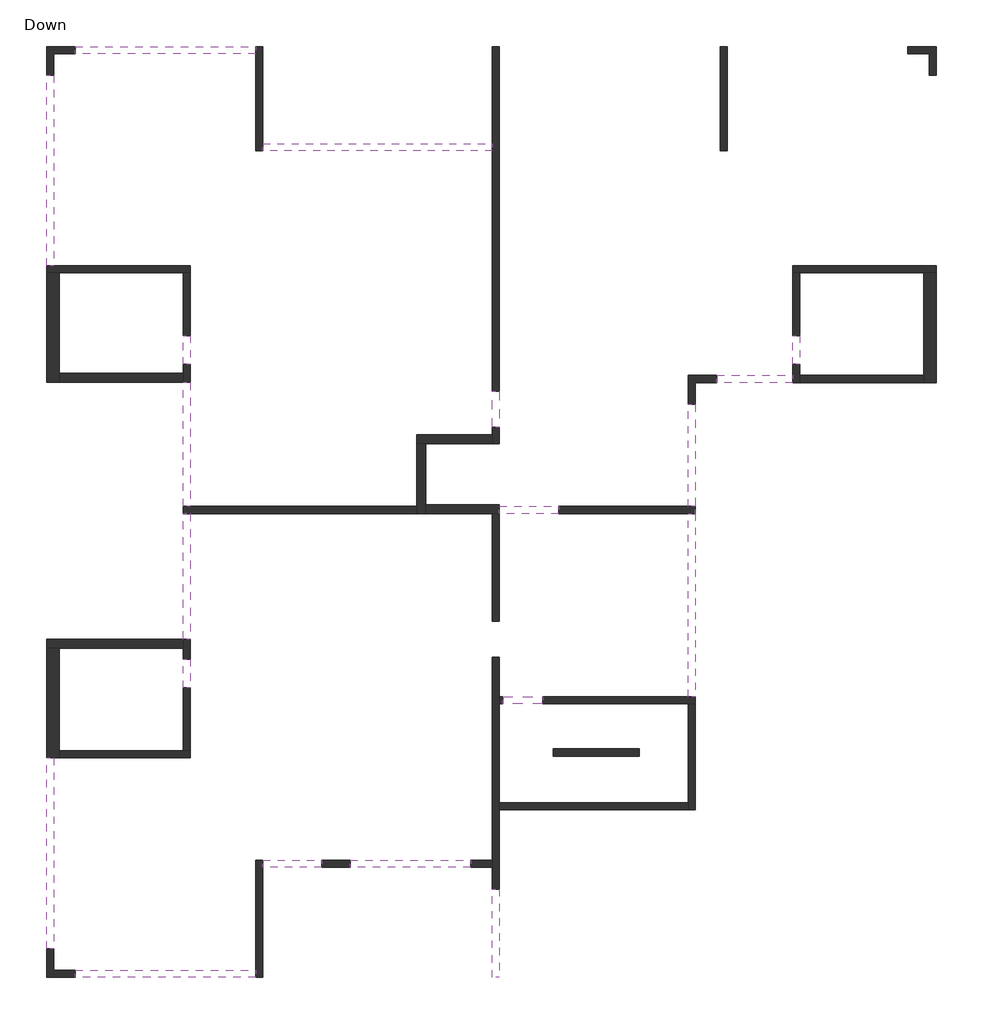
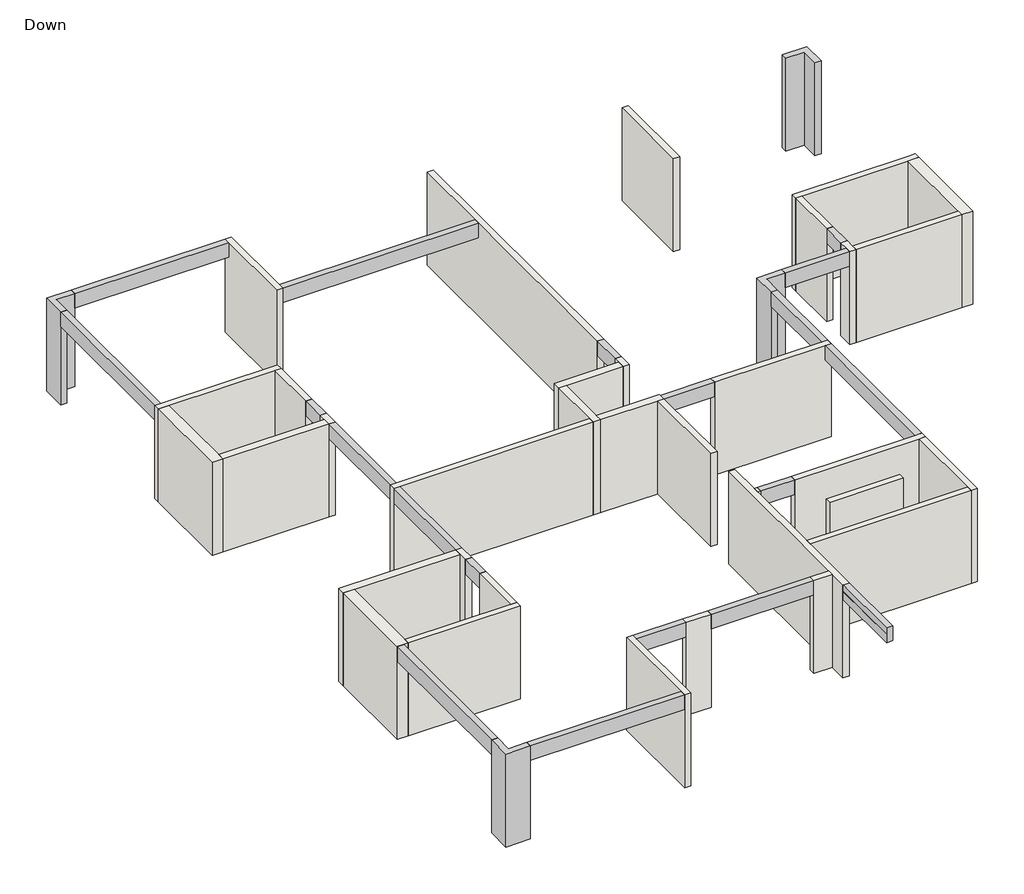
# One storey: 34 walls, 19 beams, 4 columns.
"""IFC4 building model written with IfcOpenShell, lengths in millimetres."""

from ifc_helpers import new_model, si_unit, frame, origin, origin_with_axes, place, context, project, spatial, polyline, outline, extrude, faceted_brep, element, save

model = new_model("IFC4")

# Units and contexts
model_context = context("Model", 3, world=origin())
ifc_project = project(units=[si_unit("LENGTHUNIT", "METRE", prefix="MILLI")], contexts=[model_context])

# Site, building, storey
site = spatial("IfcSite", under=ifc_project)
building = spatial("IfcBuilding", under=site)
storey = spatial("IfcBuildingStorey", under=building, Name="Down", Elevation=0.0)

# Beams
placement = place(None, origin())
element("IfcBeam", 1, ObjectType="Concrete Rectengular Beam : 20/50", at=placement, inside=storey, context=model_context, shape_type="Brep", body=[
    faceted_brep([(77.2469476, 12575.8954895, 3200.0), (77.2469476, 12375.8954895, 3200.0), (5096.9607967, 12375.8954895, 3200.0), (5096.9607967, 12575.8954895, 3200.0), (77.2469476, 12375.8954895, 2700.0), (5096.9607967, 12375.8954895, 2700.0), (5096.9607967, 12375.8954895, 2980.0), (77.2469476, 12575.8954895, 2700.0), (5096.9607967, 12575.8954895, 2700.0)], [[[0, 1, 2, 3]], [[1, 4, 5, 6, 2]], [[4, 7, 8, 5]], [[7, 0, 3, 8]], [[1, 0, 7, 4]], [[3, 2, 6, 5, 8]]]),
])
element("IfcBeam", 2, ObjectType="Concrete Rectengular Beam : 20/50", at=placement, inside=storey, context=model_context, shape_type="Brep", body=[
    faceted_brep([(-522.7530524, 11775.8954895, 3200.0), (-722.7530524, 11775.8954895, 3200.0), (-722.7530524, 6476.2289939, 3200.0), (-522.7530524, 6476.2289939, 3200.0), (-722.7530524, 11775.8954895, 2700.0), (-722.7530524, 6476.2289939, 2700.0), (-522.7530524, 11775.8954895, 2700.0), (-522.7530524, 6476.2289939, 2700.0), (-522.7530524, 6476.2289939, 2980.0)], [[[0, 1, 2, 3]], [[1, 4, 5, 2]], [[4, 6, 7, 5]], [[6, 0, 3, 8, 7]], [[1, 0, 6, 4]], [[3, 2, 5, 7, 8]]]),
])
element("IfcBeam", 3, ObjectType="Concrete Rectengular Beam : 20/50", at=placement, inside=storey, context=model_context, shape_type="Brep", body=[
    faceted_brep([(5296.9607967, 9676.3316106, 3200.0), (11679.1824488, 9676.3316106, 3200.0), (11679.1824488, 9876.3316106, 3200.0), (5296.9607967, 9876.3316106, 3200.0), (5296.9607967, 9676.3316106, 2700.0), (11679.1824488, 9676.3316106, 2700.0), (11679.1824488, 9676.3316106, 2980.0), (5296.9607967, 9876.3316106, 2700.0), (11679.1824488, 9876.3316106, 2700.0), (5296.9607967, 9876.3316106, 2980.0), (11679.1824488, 9876.3316106, 2980.0)], [[[0, 1, 2, 3]], [[1, 0, 4, 5, 6]], [[4, 7, 8, 5]], [[7, 9, 3, 2, 10, 8]], [[0, 3, 9, 7, 4]], [[2, 1, 6, 5, 8, 10]]]),
])
element("IfcBeam", 4, ObjectType="Concrete Rectengular Beam : 20/50", at=placement, inside=storey, context=model_context, shape_type="Brep", body=[
    faceted_brep([(17929.3735672, 3423.845178, 3200.0), (17929.3735672, 3223.845178, 3200.0), (20041.5682877, 3223.845178, 3200.0), (20041.5682877, 3423.845178, 3200.0), (17929.3735672, 3423.845178, 2700.0), (20041.5682877, 3423.845178, 2980.0), (20041.5682877, 3423.845178, 2700.0), (17929.3735672, 3223.845178, 2700.0), (20041.5682877, 3223.845178, 2700.0)], [[[0, 1, 2, 3]], [[4, 0, 3, 5, 6]], [[7, 4, 6, 8]], [[1, 7, 8, 2]], [[1, 0, 4, 7]], [[3, 2, 8, 6, 5]]]),
])
element("IfcBeam", 5, ObjectType="Concrete Rectengular Beam : 20/50", at=placement, inside=storey, context=model_context, shape_type="Brep", body=[
    faceted_brep([(17329.3735672, -420.2820374, 3200.0), (17329.3735672, 2623.845178, 3200.0), (17129.3735672, 2623.845178, 3200.0), (17129.3735672, -220.2820374, 3200.0), (17325.9243678, -220.2820374, 3200.0), (17325.9243678, -420.2820374, 3200.0), (17129.3735672, 2623.845178, 2700.0), (17129.3735672, -220.2820374, 2700.0), (17129.3735672, -220.2820374, 2980.0), (17329.3735672, 2623.845178, 2700.0), (17329.3735672, -420.2820374, 2700.0), (17325.9243678, -420.2820374, 2700.0), (17325.9243678, -220.2820374, 2700.0)], [[[0, 1, 2, 3, 4, 5]], [[2, 6, 7, 8, 3]], [[9, 10, 11, 12, 7, 6]], [[0, 10, 9, 1]], [[10, 0, 5, 11]], [[2, 1, 9, 6]], [[12, 4, 3, 8, 7]], [[4, 12, 11, 5]]]),
])
element("IfcBeam", 6, ObjectType="Concrete Rectengular Beam : 20/50", at=placement, inside=storey, context=model_context, shape_type="Brep", body=[
    faceted_brep([(3076.7966099, -219.230216, 3200.0), (3276.7966099, -219.230216, 3200.0), (3276.7966099, 3229.5640375, 3200.0), (3076.7966099, 3229.5640375, 3200.0), (3076.7966099, -219.230216, 2700.0), (3076.7966099, 3229.5640375, 2700.0), (3276.7966099, -219.230216, 2700.0), (3276.7966099, 3229.5640375, 2700.0), (3276.7966099, -219.230216, 2980.0)], [[[0, 1, 2, 3]], [[4, 0, 3, 5]], [[6, 4, 5, 7]], [[1, 8, 6, 7, 2]], [[1, 0, 4, 6, 8]], [[3, 2, 7, 5]]]),
])
element("IfcBeam", 7, ObjectType="Concrete Rectengular Beam : 20/50", at=placement, inside=storey, context=model_context, shape_type="Brep", body=[
    faceted_brep([(3276.7966099, -419.230216, 3200.0), (3076.7966099, -419.230216, 3200.0), (3076.7966099, -3919.8715705, 3200.0), (3276.7966099, -3919.8715705, 3200.0), (3076.7966099, -419.230216, 2700.0), (3076.7966099, -3919.8715705, 2700.0), (3276.7966099, -419.230216, 2700.0), (3276.7966099, -3919.8715705, 2700.0), (3276.7966099, -419.230216, 2980.0)], [[[0, 1, 2, 3]], [[1, 4, 5, 2]], [[4, 6, 7, 5]], [[6, 8, 0, 3, 7]], [[1, 0, 8, 6, 4]], [[3, 2, 5, 7]]]),
])
element("IfcBeam", 8, ObjectType="Concrete Rectengular Beam : 20/50", at=placement, inside=storey, context=model_context, shape_type="Brep", body=[
    faceted_brep([(17329.3735672, -420.2820374, 3200.0), (17325.9243678, -420.2820374, 3200.0), (17129.3735672, -420.2820374, 3200.0), (17129.3735672, -5519.9228789, 3200.0), (17329.3735672, -5519.9228789, 3200.0), (17129.3735672, -420.2820374, 2980.0), (17129.3735672, -420.2820374, 2700.0), (17129.3735672, -5519.9228789, 2700.0), (17129.3735672, -5519.9228789, 2980.0), (17325.9243678, -420.2820374, 2700.0), (17329.3735672, -420.2820374, 2700.0), (17329.3735672, -5519.9228789, 2700.0)], [[[0, 1, 2, 3, 4]], [[2, 5, 6, 7, 8, 3]], [[6, 9, 10, 11, 7]], [[10, 0, 4, 11]], [[2, 1, 0, 10, 9, 6, 5]], [[4, 3, 8, 7, 11]]]),
])
element("IfcBeam", 9, ObjectType="Concrete Rectengular Beam : 20/50", at=placement, inside=storey, context=model_context, shape_type="SweptSolid", body=[
    extrude(outline(polyline([(2700.0, 11678.1306274), (2700.0, 11878.1306274), (3200.0, 11878.1306274), (3200.0, 11683.1306274), (2980.0, 11683.1306274), (2980.0, 11678.1306274), (2700.0, 11678.1306274)])), frame((0.0, -13330.359, 0.0), z_axis=(0.0, 1.0, 0.0), x_axis=(0.0, 0.0, 1.0)), (0.0, 0.0, 1.0), 2460.0),
])
element("IfcBeam", 10, ObjectType="Concrete Rectengular Beam : 20/50", at=placement, inside=storey, context=model_context, shape_type="SweptSolid", body=[
    extrude(outline(polyline([(11078.1049732, -10069.2815244), (11078.1049732, -10269.2815244), (7729.8494576, -10269.2815244), (7729.8494576, -10069.2815244), (11078.1049732, -10069.2815244)])), frame((0.0, 0.0, 2700.0), z_axis=(0.0, 0.0, 1.0), x_axis=(1.0, 0.0, 0.0)), (0.0, 0.0, 1.0), 500.0),
])
element("IfcBeam", 11, ObjectType="Concrete Rectengular Beam : 20/50", at=placement, inside=storey, context=model_context, shape_type="Brep", body=[
    faceted_brep([(5300.1419152, -10069.2815244, 3200.0), (5300.1419152, -10269.2815244, 3200.0), (6929.8238034, -10269.2815244, 3200.0), (6929.8238034, -10069.2815244, 3200.0), (5300.1419152, -10069.2815244, 2700.0), (6929.8238034, -10069.2815244, 2700.0), (5300.1419152, -10269.2815244, 2700.0), (6929.8238034, -10269.2815244, 2700.0), (5300.1419152, -10269.2815244, 2980.0)], [[[0, 1, 2, 3]], [[4, 0, 3, 5]], [[6, 4, 5, 7]], [[1, 8, 6, 7, 2]], [[1, 0, 4, 6, 8]], [[3, 2, 7, 5]]]),
])
element("IfcBeam", 12, ObjectType="Concrete Rectengular Beam : 20/50", at=placement, inside=storey, context=model_context, shape_type="Brep", body=[
    faceted_brep([(77.2469476, -13130.7628896, 3200.0), (77.2469476, -13330.7628896, 3200.0), (5100.1419152, -13330.7628896, 3200.0), (5100.1419152, -13130.7628896, 3200.0), (77.2469476, -13130.7628896, 2700.0), (5100.1419152, -13130.7628896, 2980.0), (5100.1419152, -13130.7628896, 2700.0), (77.2469476, -13330.7628896, 2700.0), (5100.1419152, -13330.7628896, 2700.0)], [[[0, 1, 2, 3]], [[4, 0, 3, 5, 6]], [[7, 4, 6, 8]], [[1, 7, 8, 2]], [[1, 0, 4, 7]], [[3, 2, 8, 6, 5]]]),
])
element("IfcBeam", 13, ObjectType="Concrete Rectengular Beam : 20/50", at=placement, inside=storey, context=model_context, shape_type="Brep", body=[
    faceted_brep([(-722.7530524, -12530.7628896, 3200.0), (-522.7530524, -12530.7628896, 3200.0), (-522.7530524, -7221.5647465, 3200.0), (-722.7530524, -7221.5647465, 3200.0), (-522.7530524, -12530.7628896, 2700.0), (-522.7530524, -7221.5647465, 2700.0), (-522.7530524, -7221.5647465, 2980.0), (-722.7530524, -12530.7628896, 2700.0), (-722.7530524, -7221.5647465, 2700.0)], [[[0, 1, 2, 3]], [[1, 4, 5, 6, 2]], [[4, 7, 8, 5]], [[7, 0, 3, 8]], [[1, 0, 7, 4]], [[3, 2, 6, 5, 8]]]),
])
element("IfcBeam", 14, ObjectType="Concrete Rectengular Beam : 20/50", at=placement, inside=storey, context=model_context, shape_type="Brep", body=[
    faceted_brep([(11878.1306274, -220.2820374, 3200.0), (11878.1306274, -419.230216, 3200.0), (11878.1306274, -420.2820374, 3200.0), (13528.9772154, -420.2820374, 3200.0), (13528.9772154, -220.2820374, 3200.0), (11879.1824488, -220.2820374, 3200.0), (11878.1306274, -220.2820374, 2700.0), (13528.9772154, -220.2820374, 2700.0), (11878.1306274, -420.2820374, 2700.0), (13528.9772154, -420.2820374, 2700.0), (11878.1306274, -420.2820374, 2980.0)], [[[0, 1, 2, 3, 4, 5]], [[6, 0, 5, 4, 7]], [[8, 6, 7, 9]], [[2, 10, 8, 9, 3]], [[8, 10, 2, 1, 0, 6]], [[4, 3, 9, 7]]]),
])
element("IfcBeam", 15, ObjectType="Concrete Rectengular Beam : 20/50", at=placement, inside=storey, context=model_context, shape_type="SweptSolid", body=[
    extrude(outline(polyline([(11679.1824488, 2979.8205793), (11879.1824488, 2979.8205793), (11879.1824488, 1976.6138066), (11679.1824488, 1976.6138066), (11679.1824488, 2979.8205793)])), frame((0.0, 0.0, 2700.0), z_axis=(0.0, 0.0, 1.0), x_axis=(1.0, 0.0, 0.0)), (0.0, 0.0, 1.0), 500.0),
])
element("IfcBeam", 16, ObjectType="Concrete Rectengular Beam : 20/50", at=placement, inside=storey, context=model_context, shape_type="Brep", body=[
    faceted_brep([(11979.7211866, -5519.9228789, 3200.0), (11979.7211866, -5719.9228789, 3200.0), (13080.2855786, -5719.9228789, 3200.0), (13080.2855786, -5519.9228789, 3200.0), (11979.7211866, -5519.9228789, 2700.0), (13080.2855786, -5519.9228789, 2700.0), (11979.7211866, -5719.9228789, 2700.0), (13080.2855786, -5719.9228789, 2700.0), (13080.2855786, -5719.9228789, 2980.0)], [[[0, 1, 2, 3]], [[4, 0, 3, 5]], [[6, 4, 5, 7]], [[1, 6, 7, 8, 2]], [[1, 0, 4, 6]], [[3, 2, 8, 7, 5]]]),
])
element("IfcBeam", 17, ObjectType="Concrete Rectengular Beam : 20/50", at=placement, inside=storey, context=model_context, shape_type="SweptSolid", body=[
    extrude(outline(polyline([(3076.7966099, -4470.1537665), (3276.7966099, -4470.1537665), (3276.7966099, -5270.1794207), (3076.7966099, -5270.1794207), (3076.7966099, -4470.1537665)])), frame((0.0, 0.0, 2700.0), z_axis=(0.0, 0.0, 1.0), x_axis=(1.0, 0.0, 0.0)), (0.0, 0.0, 1.0), 500.0),
])
element("IfcBeam", 18, ObjectType="Concrete Rectengular Beam : 20/50", at=placement, inside=storey, context=model_context, shape_type="SweptSolid", body=[
    extrude(outline(polyline([(3276.7966099, 3729.0509538), (3076.7966099, 3729.0509538), (3076.7966099, 4529.076608), (3276.7966099, 4529.076608), (3276.7966099, 3729.0509538)])), frame((0.0, 0.0, 2700.0), z_axis=(0.0, 0.0, 1.0), x_axis=(1.0, 0.0, 0.0)), (0.0, 0.0, 1.0), 500.0),
])
element("IfcBeam", 19, ObjectType="Concrete Rectengular Beam : 20/50", at=placement, inside=storey, context=model_context, shape_type="SweptSolid", body=[
    extrude(outline(polyline([(20241.5682877, 3729.0509538), (20041.5682877, 3729.0509538), (20041.5682877, 4529.076608), (20241.5682877, 4529.076608), (20241.5682877, 3729.0509538)])), frame((0.0, 0.0, 2700.0), z_axis=(0.0, 0.0, 1.0), x_axis=(1.0, 0.0, 0.0)), (0.0, 0.0, 1.0), 500.0),
])

# Columns
element("IfcColumn", 20, ObjectType="L Column : 80/80/20/20", at=placement, inside=storey, context=model_context, shape_type="Brep", body=[
    faceted_brep([(-722.7530524, 12575.8954895, 0.0), (77.2469476, 12575.8954895, 0.0), (77.2469476, 12375.8954895, 0.0), (-522.7530524, 12375.8954895, 0.0), (-522.7530524, 11775.8954895, 0.0), (-722.7530524, 11775.8954895, 0.0), (-722.7530524, 12575.8954895, 3200.0), (77.2469476, 12575.8954895, 3200.0), (77.2469476, 12375.8954895, 3200.0), (-522.7530524, 12375.8954895, 3200.0), (-522.7530524, 12375.8954895, 2980.0), (-522.7530524, 11775.8954895, 3200.0), (-722.7530524, 11775.8954895, 3200.0)], [[[0, 1, 2, 3, 4, 5]], [[6, 7, 1, 0]], [[7, 8, 2, 1]], [[8, 9, 10, 3, 2]], [[9, 11, 4, 3, 10]], [[11, 12, 5, 4]], [[12, 6, 0, 5]], [[6, 12, 11, 9, 8, 7]]]),
])
element("IfcColumn", 21, ObjectType="L Column : 80/80/20/20", at=placement, inside=storey, context=model_context, shape_type="Brep", body=[
    faceted_brep([(24041.1179501, 12575.8954895, 0.0), (24041.1179501, 11775.8954895, 0.0), (23841.1179501, 11775.8954895, 0.0), (23841.1179501, 12375.8954895, 0.0), (23241.1179501, 12375.8954895, 0.0), (23241.1179501, 12575.8954895, 0.0), (24041.1179501, 12575.8954895, 3200.0), (23241.1179501, 12575.8954895, 3200.0), (23241.1179501, 12375.8954895, 3200.0), (23841.1179501, 12375.8954895, 2980.0), (23841.1179501, 12375.8954895, 3200.0), (23841.1179501, 11775.8954895, 3200.0), (24041.1179501, 11775.8954895, 3200.0)], [[[0, 1, 2, 3, 4, 5]], [[6, 0, 5, 7]], [[7, 5, 4, 8]], [[8, 4, 3, 9, 10]], [[10, 9, 3, 2, 11]], [[11, 2, 1, 12]], [[12, 1, 0, 6]], [[6, 7, 8, 10, 11, 12]]]),
])
element("IfcColumn", 22, ObjectType="L Column : 80/80/20/20", at=placement, inside=storey, context=model_context, shape_type="Brep", body=[
    faceted_brep([(17129.3735672, 3423.845178, 0.0), (17929.3735672, 3423.845178, 0.0), (17929.3735672, 3223.845178, 0.0), (17329.3735672, 3223.845178, 0.0), (17329.3735672, 2623.845178, 0.0), (17129.3735672, 2623.845178, 0.0), (17129.3735672, 3423.845178, 3200.0), (17929.3735672, 3423.845178, 3200.0), (17129.3735672, 3423.845178, 2980.0), (17929.3735672, 3223.845178, 3200.0), (17329.3735672, 3223.845178, 3200.0), (17329.3735672, 2623.845178, 3200.0), (17129.3735672, 2623.845178, 3200.0)], [[[0, 1, 2, 3, 4, 5]], [[6, 7, 1, 0, 8]], [[7, 9, 2, 1]], [[9, 10, 3, 2]], [[10, 11, 4, 3]], [[11, 12, 5, 4]], [[12, 6, 8, 0, 5]], [[6, 12, 11, 10, 9, 7]]]),
])
element("IfcColumn", 23, ObjectType="L Column : 80/80/20/20", at=placement, inside=storey, context=model_context, shape_type="Brep", body=[
    faceted_brep([(-722.7530524, -13330.7628896, 0.0), (-722.7530524, -12530.7628896, 0.0), (-522.7530524, -12530.7628896, 0.0), (-522.7530524, -13130.7628896, 0.0), (77.2469476, -13130.7628896, 0.0), (77.2469476, -13330.7628896, 0.0), (-722.7530524, -13330.7628896, 3200.0), (-722.7530524, -12530.7628896, 3200.0), (-522.7530524, -12530.7628896, 3200.0), (-522.7530524, -13130.7628896, 3200.0), (-522.7530524, -13130.7628896, 2980.0), (77.2469476, -13130.7628896, 3200.0), (77.2469476, -13330.7628896, 3200.0)], [[[0, 1, 2, 3, 4, 5]], [[6, 7, 1, 0]], [[7, 8, 2, 1]], [[8, 9, 10, 3, 2]], [[9, 11, 4, 3, 10]], [[11, 12, 5, 4]], [[12, 6, 0, 5]], [[6, 12, 11, 9, 8, 7]]]),
])

# Walls
element("IfcWall", 24, ObjectType="20", at=placement, inside=storey, context=model_context, shape_type="Brep", body=[
    faceted_brep([(3276.7966099, 6476.2289939, 0.0), (-723.331661, 6476.2289939, 0.0), (-723.331661, 6476.2289939, 3200.0), (-722.7530524, 6476.2289939, 3200.0), (-522.7530524, 6476.2289939, 3200.0), (3276.7966099, 6476.2289939, 3200.0), (3276.7966099, 6476.2289939, 2980.0), (3276.7966099, 6276.2289939, 0.0), (3276.7966099, 6276.2289939, 3200.0), (3076.7966099, 6276.2289939, 3200.0), (-373.331661, 6276.2289939, 3200.0), (-723.331661, 6276.2289939, 3200.0), (-723.331661, 6276.2289939, 0.0), (-373.331661, 6276.2289939, 0.0), (3076.7966099, 6276.2289939, 0.0)], [[[0, 1, 2, 3, 4, 5, 6]], [[7, 8, 9, 10, 11, 12, 13, 14]], [[1, 0, 7, 14, 13, 12]], [[5, 4, 3, 2, 11, 10, 9, 8]], [[2, 1, 12, 11]], [[0, 6, 5, 8, 7]]]),
])
element("IfcWall", 25, ObjectType="20", at=placement, inside=storey, context=model_context, shape_type="Brep", body=[
    faceted_brep([(3276.7966099, 3229.5640375, 0.0), (3276.7966099, 3729.0509538, 0.0), (3276.7966099, 3729.0509538, 2700.0), (3276.7966099, 3729.0509538, 3200.0), (3276.7966099, 3229.5640375, 3200.0), (3276.7966099, 3229.5640375, 2700.0), (3076.7966099, 3229.5640375, 0.0), (3076.7966099, 3229.5640375, 2700.0), (3076.7966099, 3229.5640375, 3200.0), (3076.7966099, 3479.5640375, 3200.0), (3076.7966099, 3729.0509538, 3200.0), (3076.7966099, 3729.0509538, 2700.0), (3076.7966099, 3729.0509538, 0.0), (3076.7966099, 3479.5640375, 0.0)], [[[0, 1, 2, 3, 4, 5]], [[6, 7, 8, 9, 10, 11, 12, 13]], [[1, 0, 6, 13, 12]], [[3, 2, 1, 12, 11, 10]], [[4, 3, 10, 9, 8]], [[0, 5, 4, 8, 7, 6]]]),
])
element("IfcWall", 26, ObjectType="20", at=placement, inside=storey, context=model_context, shape_type="Brep", body=[
    faceted_brep([(3276.7966099, 4529.076608, 0.0), (3276.7966099, 6276.2289939, 0.0), (3276.7966099, 6276.2289939, 3200.0), (3276.7966099, 4529.076608, 3200.0), (3276.7966099, 4529.076608, 2700.0), (3076.7966099, 4529.076608, 0.0), (3076.7966099, 4529.076608, 2700.0), (3076.7966099, 4529.076608, 3200.0), (3076.7966099, 6276.2289939, 3200.0), (3076.7966099, 6276.2289939, 2980.0), (3076.7966099, 6276.2289939, 0.0)], [[[0, 1, 2, 3, 4]], [[5, 6, 7, 8, 9, 10]], [[1, 0, 5, 10]], [[3, 2, 8, 7]], [[0, 4, 3, 7, 6, 5]], [[2, 1, 10, 9, 8]]]),
])
element("IfcWall", 27, ObjectType="20", at=placement, inside=storey, context=model_context, shape_type="Brep", body=[
    faceted_brep([(5296.9607967, 9676.3316106, 0.0), (5296.9607967, 12575.8954895, 0.0), (5296.9607967, 12575.8954895, 2980.0), (5296.9607967, 12575.8954895, 3200.0), (5296.9607967, 9876.3316106, 3200.0), (5296.9607967, 9676.3316106, 3200.0), (5096.9607967, 9676.3316106, 0.0), (5096.9607967, 9676.3316106, 2980.0), (5096.9607967, 9676.3316106, 3200.0), (5096.9607967, 12375.8954895, 3200.0), (5096.9607967, 12575.8954895, 3200.0), (5096.9607967, 12575.8954895, 0.0)], [[[0, 1, 2, 3, 4, 5]], [[6, 7, 8, 9, 10, 11]], [[1, 0, 6, 11]], [[3, 2, 1, 11, 10]], [[5, 4, 3, 10, 9, 8]], [[0, 5, 8, 7, 6]]]),
])
element("IfcWall", 28, ObjectType="20", at=placement, inside=storey, context=model_context, shape_type="Brep", body=[
    faceted_brep([(11679.1824488, 12575.8954895, 0.0), (11679.1824488, 2979.8205793, 0.0), (11679.1824488, 2979.8205793, 2700.0), (11679.1824488, 2979.8205793, 3200.0), (11679.1824488, 9676.3316106, 3200.0), (11679.1824488, 9876.3316106, 3200.0), (11679.1824488, 12575.8954895, 3200.0), (11679.1824488, 12575.8954895, 2980.0), (11879.1824488, 12575.8954895, 0.0), (11879.1824488, 12575.8954895, 2980.0), (11879.1824488, 12575.8954895, 3200.0), (11879.1824488, 9876.3316106, 3200.0), (11879.1824488, 9676.3316106, 3200.0), (11879.1824488, 2979.8205793, 3200.0), (11879.1824488, 2979.8205793, 2700.0), (11879.1824488, 2979.8205793, 0.0)], [[[0, 1, 2, 3, 4, 5, 6, 7]], [[8, 9, 10, 11, 12, 13, 14, 15]], [[1, 0, 8, 15]], [[3, 2, 1, 15, 14, 13]], [[6, 5, 4, 3, 13, 12, 11, 10]], [[0, 7, 6, 10, 9, 8]]]),
])
element("IfcWall", 29, ObjectType="20", at=placement, inside=storey, context=model_context, shape_type="Brep", body=[
    faceted_brep([(11679.1824488, 1976.6138066, 0.0), (11679.1824488, 1777.9221698, 0.0), (11679.1824488, 1527.9221698, 0.0), (11679.1824488, 1527.9221698, 3200.0), (11679.1824488, 1777.9221698, 3200.0), (11679.1824488, 1976.6138066, 3200.0), (11679.1824488, 1976.6138066, 2700.0), (11879.1824488, 1976.6138066, 0.0), (11879.1824488, 1976.6138066, 2700.0), (11879.1824488, 1976.6138066, 3200.0), (11879.1824488, 1527.9221698, 3200.0), (11879.1824488, 1527.9221698, 0.0)], [[[0, 1, 2, 3, 4, 5, 6]], [[7, 8, 9, 10, 11]], [[2, 1, 0, 7, 11]], [[5, 4, 3, 10, 9]], [[0, 6, 5, 9, 8, 7]], [[3, 2, 11, 10]]]),
])
element("IfcWall", 30, ObjectType="20", at=placement, inside=storey, context=model_context, shape_type="Brep", body=[
    faceted_brep([(9579.6442241, -219.230216, 0.0), (3076.7966099, -219.230216, 0.0), (3076.7966099, -219.230216, 3200.0), (3276.7966099, -219.230216, 3200.0), (9579.6442241, -219.230216, 3200.0), (9579.6442241, -219.230216, 2980.0), (9579.6442241, -419.230216, 0.0), (9579.6442241, -419.230216, 3200.0), (3276.7966099, -419.230216, 3200.0), (3076.7966099, -419.230216, 3200.0), (3076.7966099, -419.230216, 0.0)], [[[0, 1, 2, 3, 4, 5]], [[6, 7, 8, 9, 10]], [[1, 0, 6, 10]], [[2, 1, 10, 9]], [[4, 3, 2, 9, 8, 7]], [[0, 5, 4, 7, 6]]]),
])
element("IfcWall", 31, ObjectType="20", at=placement, inside=storey, context=model_context, shape_type="Brep", body=[
    faceted_brep([(20041.5682877, 6276.2289939, 0.0), (20241.5682877, 6276.2289939, 0.0), (23691.6965586, 6276.2289939, 0.0), (24041.6965586, 6276.2289939, 0.0), (24041.6965586, 6276.2289939, 3200.0), (23691.6965586, 6276.2289939, 3200.0), (20241.5682877, 6276.2289939, 3200.0), (20041.5682877, 6276.2289939, 3200.0), (20041.5682877, 6476.2289939, 0.0), (20041.5682877, 6476.2289939, 2980.0), (20041.5682877, 6476.2289939, 3200.0), (23841.1179501, 6476.2289939, 3200.0), (24041.1179501, 6476.2289939, 3200.0), (24041.6965586, 6476.2289939, 3200.0), (24041.6965586, 6476.2289939, 0.0)], [[[0, 1, 2, 3, 4, 5, 6, 7]], [[8, 9, 10, 11, 12, 13, 14]], [[3, 2, 1, 0, 8, 14]], [[7, 6, 5, 4, 13, 12, 11, 10]], [[4, 3, 14, 13]], [[0, 7, 10, 9, 8]]]),
])
element("IfcWall", 32, ObjectType="20", at=placement, inside=storey, context=model_context, shape_type="Brep", body=[
    faceted_brep([(23691.6965586, 3423.845178, 0.0), (20241.5682877, 3423.845178, 0.0), (20241.5682877, 3423.845178, 2980.0), (20241.5682877, 3423.845178, 3200.0), (23691.6965586, 3423.845178, 3200.0), (23691.6965586, 3423.845178, 2980.0), (23691.6965586, 3223.845178, 0.0), (23691.6965586, 3223.845178, 3200.0), (20241.5682877, 3223.845178, 3200.0), (20241.5682877, 3223.845178, 0.0)], [[[0, 1, 2, 3, 4, 5]], [[6, 7, 8, 9]], [[1, 0, 6, 9]], [[4, 3, 8, 7]], [[0, 5, 4, 7, 6]], [[3, 2, 1, 9, 8]]]),
])
element("IfcWall", 33, ObjectType="20", at=placement, inside=storey, context=model_context, shape_type="Brep", body=[
    faceted_brep([(20241.5682877, 3223.845178, 0.0), (20241.5682877, 3423.845178, 0.0), (20241.5682877, 3729.0509538, 0.0), (20241.5682877, 3729.0509538, 2700.0), (20241.5682877, 3729.0509538, 3200.0), (20241.5682877, 3423.845178, 3200.0), (20241.5682877, 3223.845178, 3200.0), (20041.5682877, 3223.845178, 0.0), (20041.5682877, 3223.845178, 3200.0), (20041.5682877, 3423.845178, 3200.0), (20041.5682877, 3729.0509538, 3200.0), (20041.5682877, 3729.0509538, 2700.0), (20041.5682877, 3729.0509538, 0.0)], [[[0, 1, 2, 3, 4, 5, 6]], [[7, 8, 9, 10, 11, 12]], [[2, 1, 0, 7, 12]], [[4, 3, 2, 12, 11, 10]], [[6, 5, 4, 10, 9, 8]], [[0, 6, 8, 7]]]),
])
element("IfcWall", 34, ObjectType="20", at=placement, inside=storey, context=model_context, shape_type="Brep", body=[
    faceted_brep([(20241.5682877, 4529.076608, 0.0), (20241.5682877, 6276.2289939, 0.0), (20241.5682877, 6276.2289939, 2980.0), (20241.5682877, 6276.2289939, 3200.0), (20241.5682877, 4529.076608, 3200.0), (20241.5682877, 4529.076608, 2700.0), (20041.5682877, 4529.076608, 0.0), (20041.5682877, 4529.076608, 2700.0), (20041.5682877, 4529.076608, 3200.0), (20041.5682877, 6276.2289939, 3200.0), (20041.5682877, 6276.2289939, 0.0)], [[[0, 1, 2, 3, 4, 5]], [[6, 7, 8, 9, 10]], [[1, 0, 6, 10]], [[4, 3, 9, 8]], [[0, 5, 4, 8, 7, 6]], [[3, 2, 1, 10, 9]]]),
])
element("IfcWall", 35, ObjectType="20", at=placement, inside=storey, context=model_context, shape_type="Brep", body=[
    faceted_brep([(18221.404101, 9676.3316106, 0.0), (18221.404101, 12575.8954895, 0.0), (18221.404101, 12575.8954895, 3200.0), (18221.404101, 12375.8954895, 3200.0), (18221.404101, 9676.3316106, 3200.0), (18221.404101, 9676.3316106, 2980.0), (18021.404101, 9676.3316106, 0.0), (18021.404101, 9676.3316106, 3200.0), (18021.404101, 9876.3316106, 3200.0), (18021.404101, 12575.8954895, 3200.0), (18021.404101, 12575.8954895, 2980.0), (18021.404101, 12575.8954895, 0.0)], [[[0, 1, 2, 3, 4, 5]], [[6, 7, 8, 9, 10, 11]], [[1, 0, 6, 11]], [[2, 1, 11, 10, 9]], [[4, 3, 2, 9, 8, 7]], [[0, 5, 4, 7, 6]]]),
])
element("IfcWall", 36, ObjectType="20", at=placement, inside=storey, context=model_context, shape_type="Brep", body=[
    faceted_brep([(13528.9772154, -420.2820374, 0.0), (17325.9243678, -420.2820374, 0.0), (17325.9243678, -420.2820374, 3200.0), (17129.3735672, -420.2820374, 3200.0), (13528.9772154, -420.2820374, 3200.0), (13528.9772154, -420.2820374, 2700.0), (13528.9772154, -220.2820374, 0.0), (13528.9772154, -220.2820374, 2700.0), (13528.9772154, -220.2820374, 3200.0), (17129.3735672, -220.2820374, 3200.0), (17325.9243678, -220.2820374, 3200.0), (17325.9243678, -220.2820374, 0.0)], [[[0, 1, 2, 3, 4, 5]], [[6, 7, 8, 9, 10, 11]], [[1, 0, 6, 11]], [[2, 1, 11, 10]], [[4, 3, 2, 10, 9, 8]], [[0, 5, 4, 8, 7, 6]]]),
])
element("IfcWall", 37, ObjectType="20", at=placement, inside=storey, context=model_context, shape_type="Brep", body=[
    faceted_brep([(11678.1306274, -419.230216, 0.0), (11678.1306274, -3420.3846542, 0.0), (11678.1306274, -3420.3846542, 2980.0), (11678.1306274, -3420.3846542, 3200.0), (11678.1306274, -419.230216, 3200.0), (11678.1306274, -419.230216, 2980.0), (11878.1306274, -419.230216, 0.0), (11878.1306274, -419.230216, 3200.0), (11878.1306274, -420.2820374, 3200.0), (11878.1306274, -3420.3846542, 3200.0), (11878.1306274, -3420.3846542, 2980.0), (11878.1306274, -3420.3846542, 0.0)], [[[0, 1, 2, 3, 4, 5]], [[6, 7, 8, 9, 10, 11]], [[1, 0, 6, 11]], [[3, 2, 1, 11, 10, 9]], [[4, 3, 9, 8, 7]], [[0, 5, 4, 7, 6]]]),
])
element("IfcWall", 38, ObjectType="20", at=placement, inside=storey, context=model_context, shape_type="Brep", body=[
    faceted_brep([(11678.1306274, -4419.3584869, 0.0), (11678.1306274, -10069.2815244, 0.0), (11678.1306274, -10269.2815244, 0.0), (11678.1306274, -10870.359, 0.0), (11678.1306274, -10870.359, 2700.0), (11678.1306274, -10870.359, 2980.0), (11678.1306274, -10870.359, 3200.0), (11678.1306274, -10269.2815244, 3200.0), (11678.1306274, -10069.2815244, 3200.0), (11678.1306274, -4419.3584869, 3200.0), (11678.1306274, -4419.3584869, 2980.0), (11878.1306274, -4419.3584869, 0.0), (11878.1306274, -4419.3584869, 2980.0), (11878.1306274, -4419.3584869, 3200.0), (11878.1306274, -5519.9228789, 3200.0), (11878.1306274, -5719.9228789, 3200.0), (11878.1306274, -8469.230216, 3200.0), (11878.1306274, -8669.230216, 3200.0), (11878.1306274, -10870.359, 3200.0), (11878.1306274, -10870.359, 2700.0), (11878.1306274, -10870.359, 0.0), (11878.1306274, -8669.230216, 0.0), (11878.1306274, -8469.230216, 0.0), (11878.1306274, -5719.9228789, 0.0), (11878.1306274, -5519.9228789, 0.0), (11683.1306274, -10870.359, 3200.0)], [[[0, 1, 2, 3, 4, 5, 6, 7, 8, 9, 10]], [[11, 12, 13, 14, 15, 16, 17, 18, 19, 20, 21, 22, 23, 24]], [[3, 2, 1, 0, 11, 24, 23, 22, 21, 20]], [[6, 5, 4, 3, 20, 19, 18, 25]], [[9, 8, 7, 6, 25, 18, 17, 16, 15, 14, 13]], [[0, 10, 9, 13, 12, 11]]]),
])
element("IfcWall", 39, ObjectType="20", at=placement, inside=storey, context=model_context, shape_type="Brep", body=[
    faceted_brep([(11678.1306274, -10069.2815244, 0.0), (11078.1049732, -10069.2815244, 0.0), (11078.1049732, -10069.2815244, 2700.0), (11078.1049732, -10069.2815244, 3200.0), (11678.1306274, -10069.2815244, 3200.0), (11678.1306274, -10069.2815244, 2980.0), (11678.1306274, -10269.2815244, 0.0), (11678.1306274, -10269.2815244, 2980.0), (11678.1306274, -10269.2815244, 3200.0), (11078.1049732, -10269.2815244, 3200.0), (11078.1049732, -10269.2815244, 2700.0), (11078.1049732, -10269.2815244, 0.0)], [[[0, 1, 2, 3, 4, 5]], [[6, 7, 8, 9, 10, 11]], [[1, 0, 6, 11]], [[3, 2, 1, 11, 10, 9]], [[4, 3, 9, 8]], [[0, 5, 4, 8, 7, 6]]]),
])
element("IfcWall", 40, ObjectType="20", at=placement, inside=storey, context=model_context, shape_type="Brep", body=[
    faceted_brep([(7729.8494576, -10069.2815244, 0.0), (6929.8238034, -10069.2815244, 0.0), (6929.8238034, -10069.2815244, 2700.0), (6929.8238034, -10069.2815244, 3200.0), (7729.8494576, -10069.2815244, 3200.0), (7729.8494576, -10069.2815244, 2700.0), (7729.8494576, -10269.2815244, 0.0), (7729.8494576, -10269.2815244, 2700.0), (7729.8494576, -10269.2815244, 3200.0), (6929.8238034, -10269.2815244, 3200.0), (6929.8238034, -10269.2815244, 2700.0), (6929.8238034, -10269.2815244, 0.0)], [[[0, 1, 2, 3, 4, 5]], [[6, 7, 8, 9, 10, 11]], [[1, 0, 6, 11]], [[3, 2, 1, 11, 10, 9]], [[4, 3, 9, 8]], [[0, 5, 4, 8, 7, 6]]]),
])
element("IfcWall", 41, ObjectType="20", at=placement, inside=storey, context=model_context, shape_type="Brep", body=[
    faceted_brep([(5100.1419152, -10069.2815244, 0.0), (5100.1419152, -13330.7628896, 0.0), (5100.1419152, -13330.7628896, 3200.0), (5100.1419152, -13130.7628896, 3200.0), (5100.1419152, -10069.2815244, 3200.0), (5100.1419152, -10069.2815244, 2980.0), (5300.1419152, -10069.2815244, 0.0), (5300.1419152, -10069.2815244, 3200.0), (5300.1419152, -10269.2815244, 3200.0), (5300.1419152, -13330.359, 3200.0), (5300.1419152, -13330.7628896, 3200.0), (5300.1419152, -13330.7628896, 0.0)], [[[0, 1, 2, 3, 4, 5]], [[6, 7, 8, 9, 10, 11]], [[1, 0, 6, 11]], [[2, 1, 11, 10]], [[4, 3, 2, 10, 9, 8, 7]], [[0, 5, 4, 7, 6]]]),
])
element("IfcWall", 42, ObjectType="20", at=placement, inside=storey, context=model_context, shape_type="Brep", body=[
    faceted_brep([(11878.1306274, -5719.9228789, 0.0), (11979.7211866, -5719.9228789, 0.0), (11979.7211866, -5719.9228789, 2700.0), (11979.7211866, -5719.9228789, 3200.0), (11878.1306274, -5719.9228789, 3200.0), (11878.1306274, -5719.9228789, 2980.0), (11878.1306274, -5519.9228789, 0.0), (11878.1306274, -5519.9228789, 2980.0), (11878.1306274, -5519.9228789, 3200.0), (11979.7211866, -5519.9228789, 3200.0), (11979.7211866, -5519.9228789, 2700.0), (11979.7211866, -5519.9228789, 0.0)], [[[0, 1, 2, 3, 4, 5]], [[6, 7, 8, 9, 10, 11]], [[1, 0, 6, 11]], [[3, 2, 1, 11, 10, 9]], [[4, 3, 9, 8]], [[0, 5, 4, 8, 7, 6]]]),
])
element("IfcWall", 43, ObjectType="20", at=placement, inside=storey, context=model_context, shape_type="Brep", body=[
    faceted_brep([(13080.2855786, -5719.9228789, 0.0), (17130.1573077, -5719.9228789, 0.0), (17330.1573077, -5719.9228789, 0.0), (17330.1573077, -5719.9228789, 3200.0), (17130.1573077, -5719.9228789, 3200.0), (13080.2855786, -5719.9228789, 3200.0), (13080.2855786, -5719.9228789, 2700.0), (13080.2855786, -5519.9228789, 0.0), (13080.2855786, -5519.9228789, 2700.0), (13080.2855786, -5519.9228789, 3200.0), (17129.3735672, -5519.9228789, 3200.0), (17330.1573077, -5519.9228789, 3200.0), (17330.1573077, -5519.9228789, 0.0)], [[[0, 1, 2, 3, 4, 5, 6]], [[7, 8, 9, 10, 11, 12]], [[2, 1, 0, 7, 12]], [[5, 4, 3, 11, 10, 9]], [[0, 6, 5, 9, 8, 7]], [[3, 2, 12, 11]]]),
])
element("IfcWall", 44, ObjectType="20", at=placement, inside=storey, context=model_context, shape_type="Brep", body=[
    faceted_brep([(17130.1573077, -5719.9228789, 0.0), (17130.1573077, -8469.230216, 0.0), (17130.1573077, -8669.230216, 0.0), (17130.1573077, -8669.230216, 3200.0), (17130.1573077, -8469.230216, 3200.0), (17130.1573077, -5719.9228789, 3200.0), (17330.1573077, -5719.9228789, 0.0), (17330.1573077, -5719.9228789, 3200.0), (17330.1573077, -8669.230216, 3200.0), (17330.1573077, -8669.230216, 0.0)], [[[0, 1, 2, 3, 4, 5]], [[6, 7, 8, 9]], [[2, 1, 0, 6, 9]], [[5, 4, 3, 8, 7]], [[0, 5, 7, 6]], [[3, 2, 9, 8]]]),
])
element("IfcWall", 45, ObjectType="20", at=placement, inside=storey, context=model_context, shape_type="Brep", body=[
    faceted_brep([(17130.1573077, -8469.230216, 0.0), (11878.1306274, -8469.230216, 0.0), (11878.1306274, -8469.230216, 2980.0), (11878.1306274, -8469.230216, 3200.0), (13080.2855786, -8469.230216, 3200.0), (17130.1573077, -8469.230216, 3200.0), (17130.1573077, -8669.230216, 0.0), (17130.1573077, -8669.230216, 3200.0), (11878.1306274, -8669.230216, 3200.0), (11878.1306274, -8669.230216, 0.0)], [[[0, 1, 2, 3, 4, 5]], [[6, 7, 8, 9]], [[1, 0, 6, 9]], [[5, 4, 3, 8, 7]], [[0, 5, 7, 6]], [[3, 2, 1, 9, 8]]]),
])
element("IfcWall", 46, ObjectType="20", at=placement, inside=storey, context=model_context, shape_type="SweptSolid", body=[
    extrude(outline(polyline([(13380.8243165, -6971.8212883), (15776.668339, -6971.8212883), (15776.668339, -7171.8212883), (13380.8243165, -7171.8212883), (13380.8243165, -6971.8212883)])), origin_with_axes(), (0.0, 0.0, 1.0), 3200.0),
])
element("IfcWall", 47, ObjectType="20", at=placement, inside=storey, context=model_context, shape_type="Brep", body=[
    faceted_brep([(3076.7966099, -3919.8715705, 0.0), (3076.7966099, -4169.8715705, 0.0), (3076.7966099, -4470.1537665, 0.0), (3076.7966099, -4470.1537665, 2700.0), (3076.7966099, -4470.1537665, 3200.0), (3076.7966099, -4169.8715705, 3200.0), (3076.7966099, -3919.8715705, 3200.0), (3076.7966099, -3919.8715705, 2700.0), (3276.7966099, -3919.8715705, 0.0), (3276.7966099, -3919.8715705, 2700.0), (3276.7966099, -3919.8715705, 3200.0), (3276.7966099, -4470.1537665, 3200.0), (3276.7966099, -4470.1537665, 2700.0), (3276.7966099, -4470.1537665, 0.0)], [[[0, 1, 2, 3, 4, 5, 6, 7]], [[8, 9, 10, 11, 12, 13]], [[2, 1, 0, 8, 13]], [[4, 3, 2, 13, 12, 11]], [[6, 5, 4, 11, 10]], [[0, 7, 6, 10, 9, 8]]]),
])
element("IfcWall", 48, ObjectType="20", at=placement, inside=storey, context=model_context, shape_type="Brep", body=[
    faceted_brep([(-373.331661, -7221.5647465, 0.0), (3276.7966099, -7221.5647465, 0.0), (3276.7966099, -7221.5647465, 2980.0), (3276.7966099, -7221.5647465, 3200.0), (-373.331661, -7221.5647465, 3200.0), (-373.331661, -7021.5647465, 0.0), (-373.331661, -7021.5647465, 2980.0), (-373.331661, -7021.5647465, 3200.0), (3076.7966099, -7021.5647465, 3200.0), (3276.7966099, -7021.5647465, 3200.0), (3276.7966099, -7021.5647465, 0.0), (3076.7966099, -7021.5647465, 0.0)], [[[0, 1, 2, 3, 4]], [[5, 6, 7, 8, 9, 10, 11]], [[1, 0, 5, 11, 10]], [[4, 3, 9, 8, 7]], [[0, 4, 7, 6, 5]], [[3, 2, 1, 10, 9]]]),
])
element("IfcWall", 49, ObjectType="20", at=placement, inside=storey, context=model_context, shape_type="Brep", body=[
    faceted_brep([(3276.7966099, -7021.5647465, 0.0), (3276.7966099, -5270.1794207, 0.0), (3276.7966099, -5270.1794207, 2700.0), (3276.7966099, -5270.1794207, 3200.0), (3276.7966099, -7021.5647465, 3200.0), (3076.7966099, -7021.5647465, 0.0), (3076.7966099, -7021.5647465, 2980.0), (3076.7966099, -7021.5647465, 3200.0), (3076.7966099, -5270.1794207, 3200.0), (3076.7966099, -5270.1794207, 2700.0), (3076.7966099, -5270.1794207, 0.0)], [[[0, 1, 2, 3, 4]], [[5, 6, 7, 8, 9, 10]], [[1, 0, 5, 10]], [[3, 2, 1, 10, 9, 8]], [[4, 3, 8, 7]], [[0, 4, 7, 6, 5]]]),
])
element("IfcWall", 50, ObjectType="25", at=placement, inside=storey, context=model_context, shape_type="Brep", body=[
    faceted_brep([(-373.331661, 3229.5640375, 0.0), (3076.7966099, 3229.5640375, 0.0), (3076.7966099, 3229.5640375, 3200.0), (-373.331661, 3229.5640375, 3200.0), (-373.331661, 3479.5640375, 0.0), (-373.331661, 3479.5640375, 2980.0), (-373.331661, 3479.5640375, 3200.0), (3076.7966099, 3479.5640375, 3200.0), (3076.7966099, 3479.5640375, 2980.0), (3076.7966099, 3479.5640375, 0.0)], [[[0, 1, 2, 3]], [[4, 5, 6, 7, 8, 9]], [[1, 0, 4, 9]], [[3, 2, 7, 6]], [[0, 3, 6, 5, 4]], [[2, 1, 9, 8, 7]]]),
])
element("IfcWall", 51, ObjectType="25", at=placement, inside=storey, context=model_context, shape_type="Brep", body=[
    faceted_brep([(11679.1824488, 1777.9221698, 0.0), (9579.6442241, 1777.9221698, 0.0), (9579.6442241, 1777.9221698, 2980.0), (9579.6442241, 1777.9221698, 3200.0), (11679.1824488, 1777.9221698, 3200.0), (11679.1824488, 1777.9221698, 2980.0), (11679.1824488, 1527.9221698, 0.0), (11679.1824488, 1527.9221698, 3200.0), (9829.6442241, 1527.9221698, 3200.0), (9579.6442241, 1527.9221698, 3200.0), (9579.6442241, 1527.9221698, 0.0), (9829.6442241, 1527.9221698, 0.0)], [[[0, 1, 2, 3, 4, 5]], [[6, 7, 8, 9, 10, 11]], [[1, 0, 6, 11, 10]], [[4, 3, 9, 8, 7]], [[0, 5, 4, 7, 6]], [[3, 2, 1, 10, 9]]]),
])
element("IfcWall", 52, ObjectType="25", at=placement, inside=storey, context=model_context, shape_type="Brep", body=[
    faceted_brep([(9579.6442241, 1527.9221698, 0.0), (9579.6442241, -219.230216, 0.0), (9579.6442241, -419.230216, 0.0), (9579.6442241, -419.230216, 3200.0), (9579.6442241, -219.230216, 3200.0), (9579.6442241, 1527.9221698, 3200.0), (9829.6442241, 1527.9221698, 0.0), (9829.6442241, 1527.9221698, 3200.0), (9829.6442241, -169.230216, 3200.0), (9829.6442241, -419.230216, 3200.0), (9829.6442241, -419.230216, 0.0), (9829.6442241, -169.230216, 0.0)], [[[0, 1, 2, 3, 4, 5]], [[6, 7, 8, 9, 10, 11]], [[2, 1, 0, 6, 11, 10]], [[5, 4, 3, 9, 8, 7]], [[0, 5, 7, 6]], [[3, 2, 10, 9]]]),
])
element("IfcWall", 53, ObjectType="25", at=placement, inside=storey, context=model_context, shape_type="Brep", body=[
    faceted_brep([(9829.6442241, -419.230216, 0.0), (11678.1306274, -419.230216, 0.0), (11878.1306274, -419.230216, 0.0), (11878.1306274, -419.230216, 3200.0), (11678.1306274, -419.230216, 3200.0), (9829.6442241, -419.230216, 3200.0), (9829.6442241, -169.230216, 0.0), (9829.6442241, -169.230216, 3200.0), (11878.1306274, -169.230216, 3200.0), (11878.1306274, -169.230216, 0.0), (11878.1306274, -220.2820374, 3200.0)], [[[0, 1, 2, 3, 4, 5]], [[6, 7, 8, 9]], [[2, 1, 0, 6, 9]], [[5, 4, 3, 10, 8, 7]], [[0, 5, 7, 6]], [[3, 2, 9, 8, 10]]]),
])
element("IfcWall", 54, ObjectType="25", at=placement, inside=storey, context=model_context, shape_type="Brep", body=[
    faceted_brep([(3076.7966099, -3919.8715705, 0.0), (-723.331661, -3919.8715705, 0.0), (-723.331661, -3919.8715705, 3200.0), (3076.7966099, -3919.8715705, 3200.0), (3076.7966099, -4169.8715705, 0.0), (3076.7966099, -4169.8715705, 2980.0), (3076.7966099, -4169.8715705, 3200.0), (-373.331661, -4169.8715705, 3200.0), (-723.331661, -4169.8715705, 3200.0), (-723.331661, -4169.8715705, 0.0), (-373.331661, -4169.8715705, 0.0)], [[[0, 1, 2, 3]], [[4, 5, 6, 7, 8, 9, 10]], [[1, 0, 4, 10, 9]], [[3, 2, 8, 7, 6]], [[0, 3, 6, 5, 4]], [[2, 1, 9, 8]]]),
])
element("IfcWall", 55, ObjectType="35", at=placement, inside=storey, context=model_context, shape_type="Brep", body=[
    faceted_brep([(-723.331661, 6276.2289939, 0.0), (-723.331661, 3229.5640375, 0.0), (-723.331661, 3229.5640375, 3200.0), (-723.331661, 6276.2289939, 3200.0), (-373.331661, 6276.2289939, 0.0), (-373.331661, 6276.2289939, 2980.0), (-373.331661, 6276.2289939, 3200.0), (-373.331661, 3479.5640375, 3200.0), (-373.331661, 3229.5640375, 3200.0), (-373.331661, 3229.5640375, 0.0), (-373.331661, 3479.5640375, 0.0)], [[[0, 1, 2, 3]], [[4, 5, 6, 7, 8, 9, 10]], [[1, 0, 4, 10, 9]], [[3, 2, 8, 7, 6]], [[0, 3, 6, 5, 4]], [[2, 1, 9, 8]]]),
])
element("IfcWall", 56, ObjectType="35", at=placement, inside=storey, context=model_context, shape_type="Brep", body=[
    faceted_brep([(23691.6965586, 6276.2289939, 0.0), (23691.6965586, 3423.845178, 0.0), (23691.6965586, 3223.845178, 0.0), (23691.6965586, 3223.845178, 3200.0), (23691.6965586, 3423.845178, 3200.0), (23691.6965586, 6276.2289939, 3200.0), (23691.6965586, 6276.2289939, 2980.0), (24041.6965586, 6276.2289939, 0.0), (24041.6965586, 6276.2289939, 3200.0), (24041.6965586, 3223.845178, 3200.0), (24041.6965586, 3223.845178, 0.0)], [[[0, 1, 2, 3, 4, 5, 6]], [[7, 8, 9, 10]], [[2, 1, 0, 7, 10]], [[5, 4, 3, 9, 8]], [[0, 6, 5, 8, 7]], [[3, 2, 10, 9]]]),
])
element("IfcWall", 57, ObjectType="35", at=placement, inside=storey, context=model_context, shape_type="Brep", body=[
    faceted_brep([(-723.331661, -4169.8715705, 0.0), (-723.331661, -7221.5647465, 0.0), (-723.331661, -7221.5647465, 3200.0), (-723.331661, -4169.8715705, 3200.0), (-373.331661, -4169.8715705, 0.0), (-373.331661, -4169.8715705, 2980.0), (-373.331661, -4169.8715705, 3200.0), (-373.331661, -7021.5647465, 3200.0), (-373.331661, -7221.5647465, 3200.0), (-373.331661, -7221.5647465, 0.0), (-373.331661, -7021.5647465, 0.0), (-722.7530524, -7221.5647465, 3200.0), (-522.7530524, -7221.5647465, 3200.0)], [[[0, 1, 2, 3]], [[4, 5, 6, 7, 8, 9, 10]], [[1, 0, 4, 10, 9]], [[3, 2, 11, 12, 8, 7, 6]], [[0, 3, 6, 5, 4]], [[2, 1, 9, 8, 12, 11]]]),
])

save(model, "model.ifc")

# Revit data of these elements
# Project information
#   Project Issue Date = "Issue Date"
#   Project Status = "Project Status"
#   Client Name = "לקוח"
#   Project Address = "Enter address here"
#   Project Name = "Project 027"
#   Project Number = "מספר פרויקט"
# Type "Concrete Rectengular Beam : 20/50"
#   Length [instance default] = 152.4 cm
#   b = 20 cm
#   h = 50 cm
#   Structural Material [instance default] = Concrete
#   Assembly Code = ""
# Type "L Column : 80/80/20/20"
#   Small Length = 20 cm
#   Small Depth = 20 cm
#   Depth = 80 cm
#   Length = 80 cm
#   Centroid Y = 70 cm
#   Centroid X = 10 cm
#   Structural Material [instance default] = Concrete, Cast-in-Place gray
# Type "20"
#   Layers, outside or top first: 20 cm "Concrete" (function 1)
# Type "25"
#   Layers, outside or top first: 25 cm "Concrete" (function 1)
# Type "35"
#   Layers, outside or top first: 35 cm "Concrete" (function 1)
# Element 1 (IfcBeam, "Concrete Rectengular Beam : 20/50")
#   Comments = ""
#   Mark = "B1"
#   SOFiSTiK_AMG_Comments = ""
#   SOFiSTiK_AMG_Scheduled = yes
#   SOFiSTiK_AMG_Adjusted = yes
#   Structural Material = Concrete
#   Phase Created = New Construction
#   Materials on its faces: "Concrete"
# Element 2 (IfcBeam, "Concrete Rectengular Beam : 20/50")
#   Comments = ""
#   Mark = "B2"
#   SOFiSTiK_AMG_Comments = ""
#   SOFiSTiK_AMG_Scheduled = yes
#   SOFiSTiK_AMG_Adjusted = yes
#   Structural Material = Concrete
#   Phase Created = New Construction
#   Materials on its faces: "Concrete"
# Element 3 (IfcBeam, "Concrete Rectengular Beam : 20/50")
#   Comments = ""
#   Mark = "B3"
#   SOFiSTiK_AMG_Comments = ""
#   SOFiSTiK_AMG_Scheduled = yes
#   SOFiSTiK_AMG_Adjusted = yes
#   Structural Material = Concrete
#   Phase Created = New Construction
#   Materials on its faces: "Concrete"
# Element 4 (IfcBeam, "Concrete Rectengular Beam : 20/50")
#   Comments = ""
#   Mark = "B7"
#   SOFiSTiK_AMG_Comments = ""
#   SOFiSTiK_AMG_Scheduled = yes
#   SOFiSTiK_AMG_Adjusted = yes
#   Structural Material = Concrete
#   Phase Created = New Construction
#   Materials on its faces: "Concrete"
# Element 5 (IfcBeam, "Concrete Rectengular Beam : 20/50")
#   Comments = ""
#   Mark = "B8"
#   SOFiSTiK_AMG_Comments = ""
#   SOFiSTiK_AMG_Scheduled = yes
#   SOFiSTiK_AMG_Adjusted = yes
#   Structural Material = Concrete
#   Phase Created = New Construction
#   Materials on its faces: "Concrete"
# Element 6 (IfcBeam, "Concrete Rectengular Beam : 20/50")
#   Comments = ""
#   Mark = "B9"
#   SOFiSTiK_AMG_Comments = ""
#   SOFiSTiK_AMG_Scheduled = yes
#   SOFiSTiK_AMG_Adjusted = yes
#   Structural Material = Concrete
#   Phase Created = New Construction
#   Materials on its faces: "Concrete"
# Element 7 (IfcBeam, "Concrete Rectengular Beam : 20/50")
#   Comments = ""
#   Mark = "B10"
#   SOFiSTiK_AMG_Comments = ""
#   SOFiSTiK_AMG_Scheduled = yes
#   SOFiSTiK_AMG_Adjusted = yes
#   Structural Material = Concrete
#   Phase Created = New Construction
#   Materials on its faces: "Concrete"
# Element 8 (IfcBeam, "Concrete Rectengular Beam : 20/50")
#   Comments = ""
#   Mark = "B11"
#   SOFiSTiK_AMG_Comments = ""
#   SOFiSTiK_AMG_Scheduled = yes
#   SOFiSTiK_AMG_Adjusted = yes
#   Structural Material = Concrete
#   Phase Created = New Construction
#   Materials on its faces: "Concrete"
# Element 9 (IfcBeam, "Concrete Rectengular Beam : 20/50")
#   Comments = ""
#   Mark = "B12"
#   SOFiSTiK_AMG_Comments = ""
#   SOFiSTiK_AMG_Scheduled = yes
#   SOFiSTiK_AMG_Adjusted = yes
#   Structural Material = Concrete
#   Phase Created = New Construction
#   Materials on its faces: "Concrete"
# Element 10 (IfcBeam, "Concrete Rectengular Beam : 20/50")
#   Comments = ""
#   Mark = "B13"
#   SOFiSTiK_AMG_Comments = ""
#   SOFiSTiK_AMG_Scheduled = yes
#   SOFiSTiK_AMG_Adjusted = yes
#   Structural Material = Concrete
#   Phase Created = New Construction
#   Materials on its faces: "Concrete"
# Element 11 (IfcBeam, "Concrete Rectengular Beam : 20/50")
#   Comments = ""
#   Mark = "B14"
#   SOFiSTiK_AMG_Comments = ""
#   SOFiSTiK_AMG_Scheduled = yes
#   SOFiSTiK_AMG_Adjusted = yes
#   Structural Material = Concrete
#   Phase Created = New Construction
#   Materials on its faces: "Concrete"
# Element 12 (IfcBeam, "Concrete Rectengular Beam : 20/50")
#   Comments = ""
#   Mark = "B15"
#   SOFiSTiK_AMG_Comments = ""
#   SOFiSTiK_AMG_Scheduled = yes
#   SOFiSTiK_AMG_Adjusted = yes
#   Structural Material = Concrete
#   Phase Created = New Construction
#   Materials on its faces: "Concrete"
# Element 13 (IfcBeam, "Concrete Rectengular Beam : 20/50")
#   Comments = ""
#   Mark = "B16"
#   SOFiSTiK_AMG_Comments = ""
#   SOFiSTiK_AMG_Scheduled = yes
#   SOFiSTiK_AMG_Adjusted = yes
#   Structural Material = Concrete
#   Phase Created = New Construction
#   Materials on its faces: "Concrete"
# Element 14 (IfcBeam, "Concrete Rectengular Beam : 20/50")
#   Comments = ""
#   Mark = "B17"
#   SOFiSTiK_AMG_Comments = ""
#   SOFiSTiK_AMG_Scheduled = yes
#   SOFiSTiK_AMG_Adjusted = yes
#   Structural Material = Concrete
#   Phase Created = New Construction
#   Materials on its faces: "Concrete"
# Element 15 (IfcBeam, "Concrete Rectengular Beam : 20/50")
#   Comments = ""
#   Mark = "B18"
#   SOFiSTiK_AMG_Comments = ""
#   SOFiSTiK_AMG_Scheduled = yes
#   SOFiSTiK_AMG_Adjusted = yes
#   Structural Material = Concrete
#   Phase Created = New Construction
#   Materials on its faces: "Concrete"
# Element 16 (IfcBeam, "Concrete Rectengular Beam : 20/50")
#   Comments = ""
#   Mark = "B19"
#   SOFiSTiK_AMG_Comments = ""
#   SOFiSTiK_AMG_Scheduled = yes
#   SOFiSTiK_AMG_Adjusted = yes
#   Structural Material = Concrete
#   Phase Created = New Construction
#   Materials on its faces: "Concrete"
# Element 17 (IfcBeam, "Concrete Rectengular Beam : 20/50")
#   Comments = ""
#   Mark = "B20"
#   SOFiSTiK_AMG_Comments = ""
#   SOFiSTiK_AMG_Scheduled = yes
#   SOFiSTiK_AMG_Adjusted = yes
#   Structural Material = Concrete
#   Phase Created = New Construction
#   Materials on its faces: "Concrete"
# Element 18 (IfcBeam, "Concrete Rectengular Beam : 20/50")
#   Comments = ""
#   Mark = "B21"
#   SOFiSTiK_AMG_Comments = ""
#   SOFiSTiK_AMG_Scheduled = yes
#   SOFiSTiK_AMG_Adjusted = yes
#   Structural Material = Concrete
#   Phase Created = New Construction
#   Materials on its faces: "Concrete"
# Element 19 (IfcBeam, "Concrete Rectengular Beam : 20/50")
#   Comments = ""
#   Mark = "B22"
#   SOFiSTiK_AMG_Comments = ""
#   SOFiSTiK_AMG_Scheduled = yes
#   SOFiSTiK_AMG_Adjusted = yes
#   Structural Material = Concrete
#   Phase Created = New Construction
#   Materials on its faces: "Concrete"
# Element 20 (IfcColumn, "L Column : 80/80/20/20")
#   Comments = ""
#   Mark = "C1"
#   SOFiSTiK_AMG_Comments = ""
#   SOFiSTiK_AMG_Scheduled = yes
#   SOFiSTiK_AMG_Adjusted = yes
#   Structural Material = Concrete
#   Phase Created = New Construction
# Element 21 (IfcColumn, "L Column : 80/80/20/20")
#   Comments = ""
#   Mark = "C2"
#   SOFiSTiK_AMG_Comments = ""
#   SOFiSTiK_AMG_Scheduled = yes
#   SOFiSTiK_AMG_Adjusted = yes
#   Structural Material = Concrete
#   Phase Created = New Construction
# Element 22 (IfcColumn, "L Column : 80/80/20/20")
#   Comments = ""
#   Mark = "C3"
#   SOFiSTiK_AMG_Comments = ""
#   SOFiSTiK_AMG_Scheduled = yes
#   SOFiSTiK_AMG_Adjusted = yes
#   Structural Material = Concrete
#   Phase Created = New Construction
# Element 23 (IfcColumn, "L Column : 80/80/20/20")
#   Comments = ""
#   Mark = "C4"
#   SOFiSTiK_AMG_Comments = ""
#   SOFiSTiK_AMG_Scheduled = yes
#   SOFiSTiK_AMG_Adjusted = yes
#   Structural Material = Concrete
#   Phase Created = New Construction
# Element 24 (IfcWall, "20")
#   Comments = ""
#   Mark = "W1"
#   SOFiSTiK_EdgeZones = "W1"
#   SOFiSTiK_AMG_Comments = ""
#   Top Offset = 0 cm
#   Base Offset = 0 cm
#   wall height = 320 cm
#   SOFiSTiK_AMG_Scheduled = yes
#   SOFiSTiK_AMG_Adjusted = yes
#   Phase Created = New Construction
#   Base Constraint = Down
#   Top Constraint = Typical Floor
#   Materials on its faces: "Concrete"
# Element 25 (IfcWall, "20")
#   Comments = ""
#   Mark = "W2"
#   SOFiSTiK_EdgeZones = "W2"
#   SOFiSTiK_AMG_Comments = ""
#   Top Offset = 0 cm
#   Base Offset = 0 cm
#   wall height = 320 cm
#   SOFiSTiK_AMG_Scheduled = yes
#   SOFiSTiK_AMG_Adjusted = yes
#   Phase Created = New Construction
#   Base Constraint = Down
#   Top Constraint = Typical Floor
#   Materials on its faces: "Concrete"
# Element 26 (IfcWall, "20")
#   Comments = ""
#   Mark = "W3"
#   SOFiSTiK_EdgeZones = "W3"
#   SOFiSTiK_AMG_Comments = ""
#   Top Offset = 0 cm
#   Base Offset = 0 cm
#   wall height = 320 cm
#   SOFiSTiK_AMG_Scheduled = yes
#   SOFiSTiK_AMG_Adjusted = yes
#   Phase Created = New Construction
#   Base Constraint = Down
#   Top Constraint = Typical Floor
#   Materials on its faces: "Concrete"
# Element 27 (IfcWall, "20")
#   Comments = ""
#   Mark = "W4"
#   SOFiSTiK_EdgeZones = "W4"
#   SOFiSTiK_AMG_Comments = ""
#   Top Offset = 0 cm
#   Base Offset = 0 cm
#   wall height = 320 cm
#   SOFiSTiK_AMG_Scheduled = yes
#   SOFiSTiK_AMG_Adjusted = yes
#   Phase Created = New Construction
#   Base Constraint = Down
#   Top Constraint = Typical Floor
#   Materials on its faces: "Concrete"
# Element 28 (IfcWall, "20")
#   Comments = ""
#   Mark = "W5"
#   SOFiSTiK_EdgeZones = "W5"
#   SOFiSTiK_AMG_Comments = ""
#   Top Offset = 0 cm
#   Base Offset = 0 cm
#   wall height = 320 cm
#   SOFiSTiK_AMG_Scheduled = yes
#   SOFiSTiK_AMG_Adjusted = yes
#   Phase Created = New Construction
#   Base Constraint = Down
#   Top Constraint = Typical Floor
#   Materials on its faces: "Concrete"
# Element 29 (IfcWall, "20")
#   Comments = ""
#   Mark = "W6"
#   SOFiSTiK_EdgeZones = "W6"
#   SOFiSTiK_AMG_Comments = ""
#   Top Offset = 0 cm
#   Base Offset = 0 cm
#   wall height = 320 cm
#   SOFiSTiK_AMG_Scheduled = yes
#   SOFiSTiK_AMG_Adjusted = yes
#   Phase Created = New Construction
#   Base Constraint = Down
#   Top Constraint = Typical Floor
#   Materials on its faces: "Concrete"
# Element 30 (IfcWall, "20")
#   Comments = ""
#   Mark = "W7"
#   SOFiSTiK_EdgeZones = "W7"
#   SOFiSTiK_AMG_Comments = ""
#   Top Offset = 0 cm
#   Base Offset = 0 cm
#   wall height = 320 cm
#   SOFiSTiK_AMG_Scheduled = yes
#   SOFiSTiK_AMG_Adjusted = yes
#   Phase Created = New Construction
